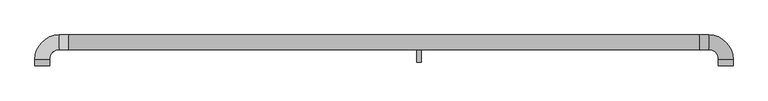
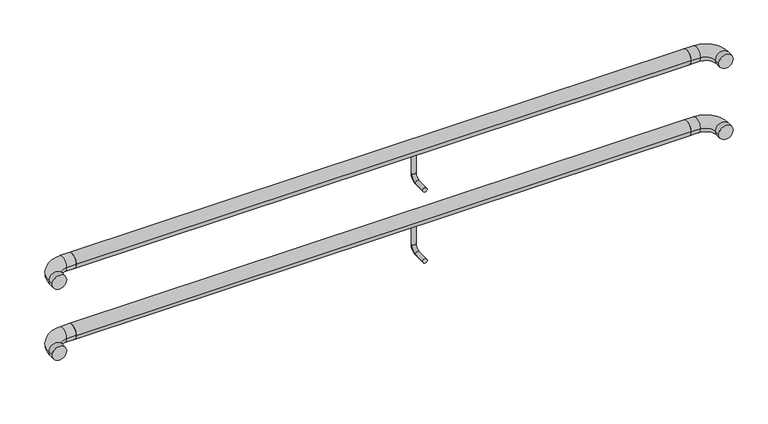
"""IFC4 building model written with IfcOpenShell, lengths in millimetres: railing geometry."""

from ifc_helpers import new_model, si_unit, point, frame, frame_2d, origin, place, context, project, spatial, circle_curve, ellipse_curve, trimmed, segment, composite_curve, outline, extrude, source, transform, mapped, element, save
from ifc_brep_helpers import plane_surface, cylinder_surface, revolved_surface, advanced_brep


def railing_7b93237a(model_context):
    return source(origin(), model_context, "Body", "SolidModel", [
        extrude(outline(composite_curve([segment(trimmed(circle_curve(frame_2d((33228.1400611, 899.0)), 21.0), [point((33249.1400611, 899.0))], [point((33207.1400611, 899.0))], False, "CARTESIAN"), True, "CONTINUOUS"), segment(trimmed(circle_curve(frame_2d((33228.1400611, 899.0)), 21.0), [point((33207.1400611, 899.0))], [point((33249.1400611, 899.0))], False, "CARTESIAN"), True, "CONTINUOUS")], self_intersect=False)), frame((9766.6129185, 0.0, 0.0), z_axis=(1.0, 0.0, 0.0), x_axis=(0.0, 1.0, 0.0)), (0.0, 0.0, 1.0), 1800.0),
        extrude(outline(composite_curve([segment(trimmed(circle_curve(frame_2d((33228.1400611, 679.0)), 21.0), [point((33249.1400611, 679.0))], [point((33207.1400611, 679.0))], False, "CARTESIAN"), True, "CONTINUOUS"), segment(trimmed(circle_curve(frame_2d((33228.1400611, 679.0)), 21.0), [point((33207.1400611, 679.0))], [point((33249.1400611, 679.0))], False, "CARTESIAN"), True, "CONTINUOUS")], self_intersect=False)), frame((9766.6129185, 0.0, 0.0), z_axis=(1.0, 0.0, 0.0), x_axis=(0.0, 1.0, 0.0)), (0.0, 0.0, 1.0), 1800.0),
        advanced_brep(
        [(10760.2629185, 33228.1900611, 658.0), (10772.9629185, 33228.1900611, 658.0), (10760.2629185, 33228.1900611, 601.05), (10772.9629185, 33228.1900611, 601.05), (10772.9629185, 33209.1400611, 582.0), (10760.2629185, 33209.1400611, 582.0), (10760.2629185, 33170.7150611, 582.0), (10772.9629185, 33170.7150611, 582.0)],
        [
            (0, 1, circle_curve(frame((10766.6129185, 33228.1900611, 658.0), z_axis=(0.0, 0.0, 1.0), x_axis=(1.0, 0.0, 0.0)), 6.35)),
            (1, 0, circle_curve(frame((10766.6129185, 33228.1900611, 658.0), z_axis=(0.0, 0.0, 1.0), x_axis=(1.0, 0.0, 0.0)), 6.35)),
            (0, 2),
            (2, 3, circle_curve(frame((10766.6129185, 33228.1900611, 601.05), z_axis=(0.0, 0.0, 1.0), x_axis=(1.0, 0.0, 0.0)), 6.35)),
            (3, 1),
            (3, 2, circle_curve(frame((10766.6129185, 33228.1900611, 601.05), z_axis=(0.0, 0.0, 1.0), x_axis=(1.0, 0.0, 0.0)), 6.35)),
            (4, 3, circle_curve(frame((10772.9629185, 33209.1400611, 601.05), z_axis=(1.0, 0.0, 0.0), x_axis=(0.0, 1.0, 0.0)), 19.05)),
            (2, 5, circle_curve(frame((10760.2629185, 33209.1400611, 601.05), z_axis=(-1.0, 0.0, 0.0), x_axis=(0.0, 1.0, 0.0)), 19.05)),
            (5, 4, circle_curve(frame((10766.6129185, 33209.1400611, 582.0), z_axis=(0.0, 1.0, 0.0), x_axis=(1.0, 0.0, 0.0)), 6.35)),
            (4, 5, circle_curve(frame((10766.6129185, 33209.1400611, 582.0), z_axis=(0.0, 1.0, 0.0), x_axis=(1.0, 0.0, 0.0)), 6.35)),
            (6, 7, circle_curve(frame((10766.6129185, 33170.7150611, 582.0), z_axis=(0.0, -1.0, 0.0), x_axis=(1.0, 0.0, 0.0)), 6.35)),
            (7, 6, circle_curve(frame((10766.6129185, 33170.7150611, 582.0), z_axis=(0.0, -1.0, 0.0), x_axis=(1.0, 0.0, 0.0)), 6.35)),
            (5, 6),
            (7, 4),
        ],
        [
            plane_surface(frame((10772.9629185, 33228.1900611, 658.0), z_axis=(0.0, 0.0, 1.0), x_axis=(0.0, -1.0, 0.0))),
            cylinder_surface(frame((10766.6129185, 33228.1900611, 658.0), z_axis=(0.0, 0.0, 1.0), x_axis=(1.0, 0.0, 0.0)), 6.35),
            revolved_surface(trimmed(ellipse_curve(frame((10766.6129185, 33228.1900611, 601.05), z_axis=(0.0, 0.0, 1.0), x_axis=(1.0, 0.0, 0.0)), 6.35, 6.35), [point((10760.2629185, 33228.1900611, 601.05))], [point((10772.9629185, 33228.1900611, 601.05))], True, "CARTESIAN"), (10766.6129185, 33209.1400611, 601.05), (-1.0, 0.0, 0.0)),
            revolved_surface(trimmed(ellipse_curve(frame((10766.6129185, 33228.1900611, 601.05), z_axis=(0.0, 0.0, 1.0), x_axis=(1.0, 0.0, 0.0)), 6.35, 6.35), [point((10772.9629185, 33228.1900611, 601.05))], [point((10760.2629185, 33228.1900611, 601.05))], True, "CARTESIAN"), (10766.6129185, 33209.1400611, 601.05), (-1.0, 0.0, 0.0)),
            plane_surface(frame((10766.6129185, 33170.7150611, 575.65), z_axis=(0.0, -1.0, 0.0), x_axis=(1.0, 0.0, 0.0))),
            cylinder_surface(frame((10766.6129185, 33209.1400611, 582.0), z_axis=(0.0, 1.0, 0.0), x_axis=(1.0, 0.0, 0.0)), 6.35),
        ],
        [
            (0, [[1, 2]]),
            (1, [[-1, 3, 4, 5]]),
            (1, [[-2, -5, 6, -3]]),
            (2, [[7, -4, 8, 9]]),
            (3, [[-8, -6, -7, 10]]),
            (4, [[11, 12]]),
            (5, [[-9, 13, -12, 14]]),
            (5, [[-10, -14, -11, -13]]),
        ],
    ),
        advanced_brep(
        [(10760.2629185, 33228.1900611, 878.0), (10772.9629185, 33228.1900611, 878.0), (10760.2629185, 33228.1900611, 821.05), (10772.9629185, 33228.1900611, 821.05), (10772.9629185, 33209.1400611, 802.0), (10760.2629185, 33209.1400611, 802.0), (10760.2629185, 33170.7150611, 802.0), (10772.9629185, 33170.7150611, 802.0)],
        [
            (0, 1, circle_curve(frame((10766.6129185, 33228.1900611, 878.0), z_axis=(0.0, 0.0, 1.0), x_axis=(1.0, 0.0, 0.0)), 6.35)),
            (1, 0, circle_curve(frame((10766.6129185, 33228.1900611, 878.0), z_axis=(0.0, 0.0, 1.0), x_axis=(1.0, 0.0, 0.0)), 6.35)),
            (0, 2),
            (2, 3, circle_curve(frame((10766.6129185, 33228.1900611, 821.05), z_axis=(0.0, 0.0, 1.0), x_axis=(1.0, 0.0, 0.0)), 6.35)),
            (3, 1),
            (3, 2, circle_curve(frame((10766.6129185, 33228.1900611, 821.05), z_axis=(0.0, 0.0, 1.0), x_axis=(1.0, 0.0, 0.0)), 6.35)),
            (4, 3, circle_curve(frame((10772.9629185, 33209.1400611, 821.05), z_axis=(1.0, 0.0, 0.0), x_axis=(0.0, 1.0, 0.0)), 19.05)),
            (2, 5, circle_curve(frame((10760.2629185, 33209.1400611, 821.05), z_axis=(-1.0, 0.0, 0.0), x_axis=(0.0, 1.0, 0.0)), 19.05)),
            (5, 4, circle_curve(frame((10766.6129185, 33209.1400611, 802.0), z_axis=(0.0, 1.0, 0.0), x_axis=(1.0, 0.0, 0.0)), 6.35)),
            (4, 5, circle_curve(frame((10766.6129185, 33209.1400611, 802.0), z_axis=(0.0, 1.0, 0.0), x_axis=(1.0, 0.0, 0.0)), 6.35)),
            (6, 7, circle_curve(frame((10766.6129185, 33170.7150611, 802.0), z_axis=(0.0, -1.0, 0.0), x_axis=(1.0, 0.0, 0.0)), 6.35)),
            (7, 6, circle_curve(frame((10766.6129185, 33170.7150611, 802.0), z_axis=(0.0, -1.0, 0.0), x_axis=(1.0, 0.0, 0.0)), 6.35)),
            (5, 6),
            (7, 4),
        ],
        [
            plane_surface(frame((10772.9629185, 33228.1900611, 878.0), z_axis=(0.0, 0.0, 1.0), x_axis=(0.0, -1.0, 0.0))),
            cylinder_surface(frame((10766.6129185, 33228.1900611, 878.0), z_axis=(0.0, 0.0, 1.0), x_axis=(1.0, 0.0, 0.0)), 6.35),
            revolved_surface(trimmed(ellipse_curve(frame((10766.6129185, 33228.1900611, 821.05), z_axis=(0.0, 0.0, 1.0), x_axis=(1.0, 0.0, 0.0)), 6.35, 6.35), [point((10760.2629185, 33228.1900611, 821.05))], [point((10772.9629185, 33228.1900611, 821.05))], True, "CARTESIAN"), (10766.6129185, 33209.1400611, 821.05), (-1.0, 0.0, 0.0)),
            revolved_surface(trimmed(ellipse_curve(frame((10766.6129185, 33228.1900611, 821.05), z_axis=(0.0, 0.0, 1.0), x_axis=(1.0, 0.0, 0.0)), 6.35, 6.35), [point((10772.9629185, 33228.1900611, 821.05))], [point((10760.2629185, 33228.1900611, 821.05))], True, "CARTESIAN"), (10766.6129185, 33209.1400611, 821.05), (-1.0, 0.0, 0.0)),
            plane_surface(frame((10766.6129185, 33170.7150611, 795.65), z_axis=(0.0, -1.0, 0.0), x_axis=(1.0, 0.0, 0.0))),
            cylinder_surface(frame((10766.6129185, 33209.1400611, 802.0), z_axis=(0.0, 1.0, 0.0), x_axis=(1.0, 0.0, 0.0)), 6.35),
        ],
        [
            (0, [[1, 2]]),
            (1, [[-1, 3, 4, 5]]),
            (1, [[-2, -5, 6, -3]]),
            (2, [[7, -4, 8, 9]]),
            (3, [[-8, -6, -7, 10]]),
            (4, [[11, 12]]),
            (5, [[-9, 13, -12, 14]]),
            (5, [[-10, -14, -11, -13]]),
        ],
    ),
        advanced_brep(
        [(11566.6129185, 33207.1900611, 679.1), (11566.6129185, 33249.1900611, 679.1), (11594.1129185, 33207.1900611, 679.1), (11594.1129185, 33249.1900611, 679.1), (11663.6129185, 33179.6900611, 679.1), (11621.6129185, 33179.6900611, 679.1), (11621.6129185, 33161.1900611, 679.1), (11663.6129185, 33161.1900611, 679.1)],
        [
            (0, 1, circle_curve(frame((11566.6129185, 33228.1900611, 679.1), z_axis=(-1.0, 0.0, 0.0), x_axis=(0.0, 1.0, 0.0)), 21.0)),
            (1, 0, circle_curve(frame((11566.6129185, 33228.1900611, 679.1), z_axis=(-1.0, 0.0, 0.0), x_axis=(0.0, 1.0, 0.0)), 21.0)),
            (0, 2),
            (2, 3, circle_curve(frame((11594.1129185, 33228.1900611, 679.1), z_axis=(-1.0, 0.0, 0.0), x_axis=(0.0, 1.0, 0.0)), 21.0)),
            (3, 1),
            (3, 2, circle_curve(frame((11594.1129185, 33228.1900611, 679.1), z_axis=(-1.0, 0.0, 0.0), x_axis=(0.0, 1.0, 0.0)), 21.0)),
            (4, 3, circle_curve(frame((11594.1129185, 33179.6900611, 679.1), z_axis=(0.0, 0.0, 1.0), x_axis=(0.0, 1.0, 0.0)), 69.5)),
            (2, 5, circle_curve(frame((11594.1129185, 33179.6900611, 679.1), z_axis=(0.0, 0.0, -1.0), x_axis=(0.0, 1.0, 0.0)), 27.5)),
            (5, 4, circle_curve(frame((11642.6129185, 33179.6900611, 679.1), z_axis=(0.0, 1.0, 0.0), x_axis=(1.0, 0.0, 0.0)), 21.0)),
            (4, 5, circle_curve(frame((11642.6129185, 33179.6900611, 679.1), z_axis=(0.0, 1.0, 0.0), x_axis=(1.0, 0.0, 0.0)), 21.0)),
            (6, 7, circle_curve(frame((11642.6129185, 33161.1900611, 679.1), z_axis=(0.0, -1.0, 0.0), x_axis=(1.0, 0.0, 0.0)), 21.0)),
            (7, 6, circle_curve(frame((11642.6129185, 33161.1900611, 679.1), z_axis=(0.0, -1.0, 0.0), x_axis=(1.0, 0.0, 0.0)), 21.0)),
            (5, 6),
            (7, 4),
        ],
        [
            plane_surface(frame((11566.6129185, 33228.1900611, 679.1), z_axis=(-1.0, 0.0, 0.0), x_axis=(0.0, 0.0, 1.0))),
            cylinder_surface(frame((11566.6129185, 33228.1900611, 679.1), z_axis=(-1.0, 0.0, 0.0), x_axis=(0.0, 1.0, 0.0)), 21.0),
            revolved_surface(trimmed(ellipse_curve(frame((11594.1129185, 33228.1900611, 679.1), z_axis=(-1.0, 0.0, 0.0), x_axis=(0.0, 1.0, 0.0)), 21.0, 21.0), [point((11594.1129185, 33207.1900611, 679.1))], [point((11594.1129185, 33249.1900611, 679.1))], True, "CARTESIAN"), (11594.1129185, 33179.6900611, 679.1), (0.0, 0.0, -1.0)),
            revolved_surface(trimmed(ellipse_curve(frame((11594.1129185, 33228.1900611, 679.1), z_axis=(-1.0, 0.0, 0.0), x_axis=(0.0, 1.0, 0.0)), 21.0, 21.0), [point((11594.1129185, 33249.1900611, 679.1))], [point((11594.1129185, 33207.1900611, 679.1))], True, "CARTESIAN"), (11594.1129185, 33179.6900611, 679.1), (0.0, 0.0, -1.0)),
            plane_surface(frame((11642.6129185, 33161.1900611, 679.1), z_axis=(0.0, -1.0, 0.0), x_axis=(0.0, 0.0, 1.0))),
            cylinder_surface(frame((11642.6129185, 33179.6900611, 679.1), z_axis=(0.0, 1.0, 0.0), x_axis=(1.0, 0.0, 0.0)), 21.0),
        ],
        [
            (0, [[1, 2]]),
            (1, [[-1, 3, 4, 5]]),
            (1, [[-2, -5, 6, -3]]),
            (2, [[7, -4, 8, 9]]),
            (3, [[-8, -6, -7, 10]]),
            (4, [[11, 12]]),
            (5, [[-9, 13, -12, 14]]),
            (5, [[-10, -14, -11, -13]]),
        ],
    ),
        advanced_brep(
        [(11566.6129185, 33207.1900611, 899.1), (11566.6129185, 33249.1900611, 899.1), (11594.1129185, 33207.1900611, 899.1), (11594.1129185, 33249.1900611, 899.1), (11663.6129185, 33179.6900611, 899.1), (11621.6129185, 33179.6900611, 899.1), (11621.6129185, 33161.1900611, 899.1), (11663.6129185, 33161.1900611, 899.1)],
        [
            (0, 1, circle_curve(frame((11566.6129185, 33228.1900611, 899.1), z_axis=(-1.0, 0.0, 0.0), x_axis=(0.0, 1.0, 0.0)), 21.0)),
            (1, 0, circle_curve(frame((11566.6129185, 33228.1900611, 899.1), z_axis=(-1.0, 0.0, 0.0), x_axis=(0.0, 1.0, 0.0)), 21.0)),
            (0, 2),
            (2, 3, circle_curve(frame((11594.1129185, 33228.1900611, 899.1), z_axis=(-1.0, 0.0, 0.0), x_axis=(0.0, 1.0, 0.0)), 21.0)),
            (3, 1),
            (3, 2, circle_curve(frame((11594.1129185, 33228.1900611, 899.1), z_axis=(-1.0, 0.0, 0.0), x_axis=(0.0, 1.0, 0.0)), 21.0)),
            (4, 3, circle_curve(frame((11594.1129185, 33179.6900611, 899.1), z_axis=(0.0, 0.0, 1.0), x_axis=(0.0, 1.0, 0.0)), 69.5)),
            (2, 5, circle_curve(frame((11594.1129185, 33179.6900611, 899.1), z_axis=(0.0, 0.0, -1.0), x_axis=(0.0, 1.0, 0.0)), 27.5)),
            (5, 4, circle_curve(frame((11642.6129185, 33179.6900611, 899.1), z_axis=(0.0, 1.0, 0.0), x_axis=(1.0, 0.0, 0.0)), 21.0)),
            (4, 5, circle_curve(frame((11642.6129185, 33179.6900611, 899.1), z_axis=(0.0, 1.0, 0.0), x_axis=(1.0, 0.0, 0.0)), 21.0)),
            (6, 7, circle_curve(frame((11642.6129185, 33161.1900611, 899.1), z_axis=(0.0, -1.0, 0.0), x_axis=(1.0, 0.0, 0.0)), 21.0)),
            (7, 6, circle_curve(frame((11642.6129185, 33161.1900611, 899.1), z_axis=(0.0, -1.0, 0.0), x_axis=(1.0, 0.0, 0.0)), 21.0)),
            (5, 6),
            (7, 4),
        ],
        [
            plane_surface(frame((11566.6129185, 33228.1900611, 899.1), z_axis=(-1.0, 0.0, 0.0), x_axis=(0.0, 0.0, 1.0))),
            cylinder_surface(frame((11566.6129185, 33228.1900611, 899.1), z_axis=(-1.0, 0.0, 0.0), x_axis=(0.0, 1.0, 0.0)), 21.0),
            revolved_surface(trimmed(ellipse_curve(frame((11594.1129185, 33228.1900611, 899.1), z_axis=(-1.0, 0.0, 0.0), x_axis=(0.0, 1.0, 0.0)), 21.0, 21.0), [point((11594.1129185, 33207.1900611, 899.1))], [point((11594.1129185, 33249.1900611, 899.1))], True, "CARTESIAN"), (11594.1129185, 33179.6900611, 899.1), (0.0, 0.0, -1.0)),
            revolved_surface(trimmed(ellipse_curve(frame((11594.1129185, 33228.1900611, 899.1), z_axis=(-1.0, 0.0, 0.0), x_axis=(0.0, 1.0, 0.0)), 21.0, 21.0), [point((11594.1129185, 33249.1900611, 899.1))], [point((11594.1129185, 33207.1900611, 899.1))], True, "CARTESIAN"), (11594.1129185, 33179.6900611, 899.1), (0.0, 0.0, -1.0)),
            plane_surface(frame((11642.6129185, 33161.1900611, 899.1), z_axis=(0.0, -1.0, 0.0), x_axis=(0.0, 0.0, 1.0))),
            cylinder_surface(frame((11642.6129185, 33179.6900611, 899.1), z_axis=(0.0, 1.0, 0.0), x_axis=(1.0, 0.0, 0.0)), 21.0),
        ],
        [
            (0, [[1, 2]]),
            (1, [[-1, 3, 4, 5]]),
            (1, [[-2, -5, 6, -3]]),
            (2, [[7, -4, 8, 9]]),
            (3, [[-8, -6, -7, 10]]),
            (4, [[11, 12]]),
            (5, [[-9, 13, -12, 14]]),
            (5, [[-10, -14, -11, -13]]),
        ],
    ),
        advanced_brep(
        [(9766.6129185, 33249.1900611, 679.1), (9766.6129185, 33207.1900611, 679.1), (9739.1129185, 33207.1900611, 679.1), (9739.1129185, 33249.1900611, 679.1), (9669.6129185, 33179.6900611, 679.1), (9711.6129185, 33179.6900611, 679.1), (9711.6129185, 33161.1900611, 679.1), (9669.6129185, 33161.1900611, 679.1)],
        [
            (0, 1, circle_curve(frame((9766.6129185, 33228.1900611, 679.1), z_axis=(1.0, 0.0, 0.0), x_axis=(0.0, -1.0, 0.0)), 21.0)),
            (1, 0, circle_curve(frame((9766.6129185, 33228.1900611, 679.1), z_axis=(1.0, 0.0, 0.0), x_axis=(0.0, -1.0, 0.0)), 21.0)),
            (1, 2),
            (2, 3, circle_curve(frame((9739.1129185, 33228.1900611, 679.1), z_axis=(1.0, 0.0, 0.0), x_axis=(0.0, -1.0, 0.0)), 21.0)),
            (3, 0),
            (3, 2, circle_curve(frame((9739.1129185, 33228.1900611, 679.1), z_axis=(1.0, 0.0, 0.0), x_axis=(0.0, -1.0, 0.0)), 21.0)),
            (4, 3, circle_curve(frame((9739.1129185, 33179.6900611, 679.1), z_axis=(0.0, 0.0, -1.0), x_axis=(0.0, 1.0, 0.0)), 69.5)),
            (2, 5, circle_curve(frame((9739.1129185, 33179.6900611, 679.1), z_axis=(0.0, 0.0, 1.0), x_axis=(0.0, 1.0, 0.0)), 27.5)),
            (5, 4, circle_curve(frame((9690.6129185, 33179.6900611, 679.1), z_axis=(0.0, 1.0, 0.0), x_axis=(1.0, 0.0, 0.0)), 21.0)),
            (4, 5, circle_curve(frame((9690.6129185, 33179.6900611, 679.1), z_axis=(0.0, 1.0, 0.0), x_axis=(1.0, 0.0, 0.0)), 21.0)),
            (5, 6),
            (6, 7, circle_curve(frame((9690.6129185, 33161.1900611, 679.1), z_axis=(0.0, 1.0, 0.0), x_axis=(1.0, 0.0, 0.0)), 21.0)),
            (7, 4),
            (7, 6, circle_curve(frame((9690.6129185, 33161.1900611, 679.1), z_axis=(0.0, 1.0, 0.0), x_axis=(1.0, 0.0, 0.0)), 21.0)),
        ],
        [
            plane_surface(frame((9766.6129185, 33228.1900611, 679.1), z_axis=(1.0, 0.0, 0.0), x_axis=(0.0, 0.0, 1.0))),
            cylinder_surface(frame((9766.6129185, 33228.1900611, 679.1), z_axis=(1.0, 0.0, 0.0), x_axis=(0.0, -1.0, 0.0)), 21.0),
            revolved_surface(trimmed(ellipse_curve(frame((9739.1129185, 33228.1900611, 679.1), z_axis=(1.0, 0.0, 0.0), x_axis=(0.0, -1.0, 0.0)), 21.0, 21.0), [point((9739.1129185, 33207.1900611, 679.1))], [point((9739.1129185, 33249.1900611, 679.1))], True, "CARTESIAN"), (9739.1129185, 33179.6900611, 679.1), (0.0, 0.0, 1.0)),
            revolved_surface(trimmed(ellipse_curve(frame((9739.1129185, 33228.1900611, 679.1), z_axis=(1.0, 0.0, 0.0), x_axis=(0.0, -1.0, 0.0)), 21.0, 21.0), [point((9739.1129185, 33249.1900611, 679.1))], [point((9739.1129185, 33207.1900611, 679.1))], True, "CARTESIAN"), (9739.1129185, 33179.6900611, 679.1), (0.0, 0.0, 1.0)),
            cylinder_surface(frame((9690.6129185, 33179.6900611, 679.1), z_axis=(0.0, 1.0, 0.0), x_axis=(1.0, 0.0, 0.0)), 21.0),
            plane_surface(frame((9690.6129185, 33161.1900611, 679.1), z_axis=(0.0, -1.0, 0.0), x_axis=(0.0, 0.0, 1.0))),
        ],
        [
            (0, [[1, 2]]),
            (1, [[-2, 3, 4, 5]]),
            (1, [[-1, -5, 6, -3]]),
            (2, [[7, -4, 8, 9]]),
            (3, [[-8, -6, -7, 10]]),
            (4, [[-9, 11, 12, 13]]),
            (4, [[-10, -13, 14, -11]]),
            (5, [[-12, -14]]),
        ],
    ),
        advanced_brep(
        [(9766.6129185, 33249.1900611, 899.1), (9766.6129185, 33207.1900611, 899.1), (9739.1129185, 33207.1900611, 899.1), (9739.1129185, 33249.1900611, 899.1), (9669.6129185, 33179.6900611, 899.1), (9711.6129185, 33179.6900611, 899.1), (9669.6129185, 33161.1900611, 899.1), (9711.6129185, 33161.1900611, 899.1)],
        [
            (0, 1, circle_curve(frame((9766.6129185, 33228.1900611, 899.1), z_axis=(1.0, 0.0, 0.0), x_axis=(0.0, -1.0, 0.0)), 21.0)),
            (1, 0, circle_curve(frame((9766.6129185, 33228.1900611, 899.1), z_axis=(1.0, 0.0, 0.0), x_axis=(0.0, -1.0, 0.0)), 21.0)),
            (1, 2),
            (2, 3, circle_curve(frame((9739.1129185, 33228.1900611, 899.1), z_axis=(1.0, 0.0, 0.0), x_axis=(0.0, -1.0, 0.0)), 21.0)),
            (3, 0),
            (3, 2, circle_curve(frame((9739.1129185, 33228.1900611, 899.1), z_axis=(1.0, 0.0, 0.0), x_axis=(0.0, -1.0, 0.0)), 21.0)),
            (4, 3, circle_curve(frame((9739.1129185, 33179.6900611, 899.1), z_axis=(0.0, 0.0, -1.0), x_axis=(0.0, 1.0, 0.0)), 69.5)),
            (2, 5, circle_curve(frame((9739.1129185, 33179.6900611, 899.1), z_axis=(0.0, 0.0, 1.0), x_axis=(0.0, 1.0, 0.0)), 27.5)),
            (5, 4, circle_curve(frame((9690.6129185, 33179.6900611, 899.1), z_axis=(0.0, 1.0, 0.0), x_axis=(1.0, 0.0, 0.0)), 21.0)),
            (4, 5, circle_curve(frame((9690.6129185, 33179.6900611, 899.1), z_axis=(0.0, 1.0, 0.0), x_axis=(1.0, 0.0, 0.0)), 21.0)),
            (6, 7, circle_curve(frame((9690.6129185, 33161.1900611, 899.1), z_axis=(0.0, -1.0, 0.0), x_axis=(1.0, 0.0, 0.0)), 21.0)),
            (7, 6, circle_curve(frame((9690.6129185, 33161.1900611, 899.1), z_axis=(0.0, -1.0, 0.0), x_axis=(1.0, 0.0, 0.0)), 21.0)),
            (5, 7),
            (6, 4),
        ],
        [
            plane_surface(frame((9766.6129185, 33228.1900611, 899.1), z_axis=(1.0, 0.0, 0.0), x_axis=(0.0, 0.0, 1.0))),
            cylinder_surface(frame((9766.6129185, 33228.1900611, 899.1), z_axis=(1.0, 0.0, 0.0), x_axis=(0.0, -1.0, 0.0)), 21.0),
            revolved_surface(trimmed(ellipse_curve(frame((9739.1129185, 33228.1900611, 899.1), z_axis=(1.0, 0.0, 0.0), x_axis=(0.0, -1.0, 0.0)), 21.0, 21.0), [point((9739.1129185, 33207.1900611, 899.1))], [point((9739.1129185, 33249.1900611, 899.1))], True, "CARTESIAN"), (9739.1129185, 33179.6900611, 899.1), (0.0, 0.0, 1.0)),
            revolved_surface(trimmed(ellipse_curve(frame((9739.1129185, 33228.1900611, 899.1), z_axis=(1.0, 0.0, 0.0), x_axis=(0.0, -1.0, 0.0)), 21.0, 21.0), [point((9739.1129185, 33249.1900611, 899.1))], [point((9739.1129185, 33207.1900611, 899.1))], True, "CARTESIAN"), (9739.1129185, 33179.6900611, 899.1), (0.0, 0.0, 1.0)),
            plane_surface(frame((9690.6129185, 33161.1900611, 899.1), z_axis=(0.0, -1.0, 0.0), x_axis=(0.0, 0.0, 1.0))),
            cylinder_surface(frame((9690.6129185, 33179.6900611, 899.1), z_axis=(0.0, 1.0, 0.0), x_axis=(1.0, 0.0, 0.0)), 21.0),
        ],
        [
            (0, [[1, 2]]),
            (1, [[-2, 3, 4, 5]]),
            (1, [[-1, -5, 6, -3]]),
            (2, [[7, -4, 8, 9]]),
            (3, [[-8, -6, -7, 10]]),
            (4, [[11, 12]]),
            (5, [[-9, 13, -11, 14]]),
            (5, [[-10, -14, -12, -13]]),
        ],
    ),
    ])


if __name__ == "__main__":
    model = new_model("IFC4")
    model_context = context("Model", 3, world=origin())
    ifc_project = project(units=[si_unit("LENGTHUNIT", "METRE", prefix="MILLI")], contexts=[model_context])
    site = spatial("IfcSite", under=ifc_project)
    building = spatial("IfcBuilding", under=site)
    placement = place(None, origin())
    railing_shape = railing_7b93237a(model_context)
    element("IfcRailing", 1, at=placement, inside=building, context=model_context, shape_type="MappedRepresentation", body=[
        mapped(railing_shape, transform((0.0, 0.0, 0.0), x_axis=(1.0, 0.0, 0.0), y_axis=(0.0, 1.0, 0.0), z_axis=(0.0, 0.0, 1.0))),
    ])
    save(model, "model.ifc")

# Revit data of these elements
# Element 1 (IfcRailing)
#   Materials on its faces: "Ferro - Pintura Esmalte"
# Materials
#   "Ferro - Pintura Esmalte": class "Pintura", colour RGB 255 255 255, transparency 0, Cost = 0
